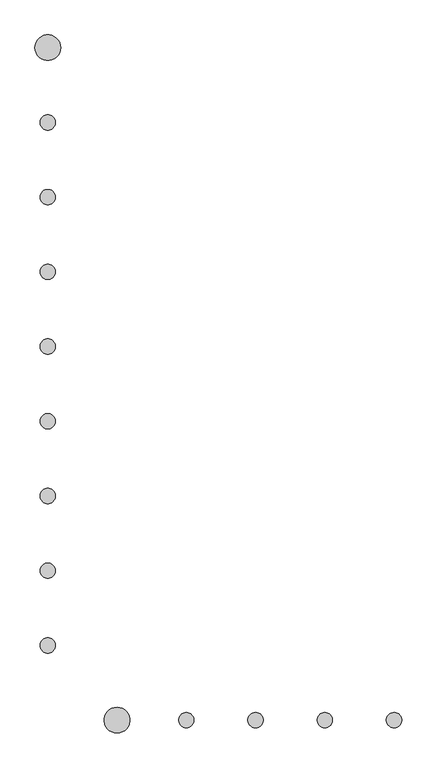
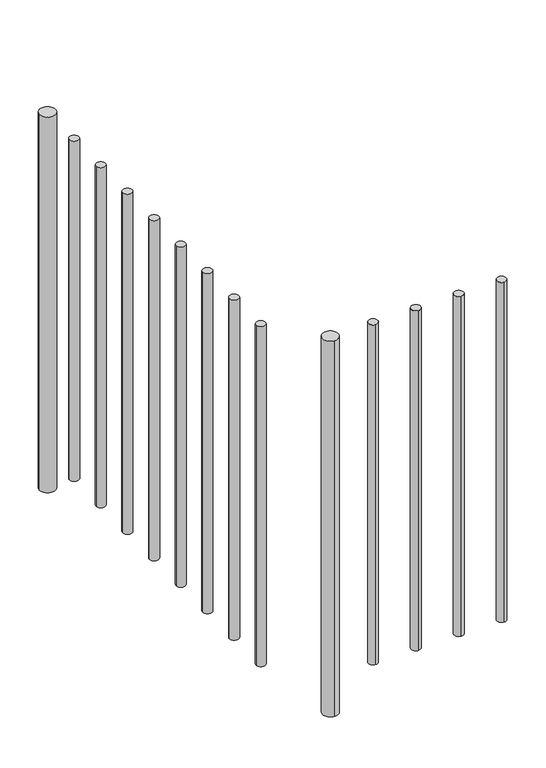
"""IFC4 building model written with IfcOpenShell, lengths in millimetres: railing geometry."""

from ifc_helpers import new_model, si_unit, point, frame, frame_2d, origin, place, context, project, spatial, circle_curve, trimmed, segment, composite_curve, outline, extrude, source, transform, mapped, element, save


def railing_35eac12f(model_context):
    return source(origin(), model_context, "Body", "SweptSolid", [
        extrude(outline(composite_curve([segment(trimmed(circle_curve(frame_2d((-2709.174449, -8163.7965465)), 12.5), [point((-2709.174449, -8176.2965465))], [point((-2709.174449, -8151.2965465))], False, "CARTESIAN"), True, "CONTINUOUS"), segment(trimmed(circle_curve(frame_2d((-2709.174449, -8163.7965465)), 12.5), [point((-2709.174449, -8151.2965465))], [point((-2709.174449, -8176.2965465))], False, "CARTESIAN"), True, "CONTINUOUS")], self_intersect=False)), frame((0.0, 0.0, 3500.0), z_axis=(0.0, 0.0, 1.0), x_axis=(1.0, 0.0, 0.0)), (0.0, 0.0, 1.0), 949.2),
        extrude(outline(composite_curve([segment(trimmed(circle_curve(frame_2d((-2822.314449, -8163.7965465)), 12.5), [point((-2822.314449, -8176.2965465))], [point((-2822.314449, -8151.2965465))], False, "CARTESIAN"), True, "CONTINUOUS"), segment(trimmed(circle_curve(frame_2d((-2822.314449, -8163.7965465)), 12.5), [point((-2822.314449, -8151.2965465))], [point((-2822.314449, -8176.2965465))], False, "CARTESIAN"), True, "CONTINUOUS")], self_intersect=False)), frame((0.0, 0.0, 3500.0), z_axis=(0.0, 0.0, 1.0), x_axis=(1.0, 0.0, 0.0)), (0.0, 0.0, 1.0), 949.2),
        extrude(outline(composite_curve([segment(trimmed(circle_curve(frame_2d((-2935.454449, -8163.7965465)), 12.5), [point((-2935.454449, -8176.2965465))], [point((-2935.454449, -8151.2965465))], False, "CARTESIAN"), True, "CONTINUOUS"), segment(trimmed(circle_curve(frame_2d((-2935.454449, -8163.7965465)), 12.5), [point((-2935.454449, -8151.2965465))], [point((-2935.454449, -8176.2965465))], False, "CARTESIAN"), True, "CONTINUOUS")], self_intersect=False)), frame((0.0, 0.0, 3500.0), z_axis=(0.0, 0.0, 1.0), x_axis=(1.0, 0.0, 0.0)), (0.0, 0.0, 1.0), 949.2),
        extrude(outline(composite_curve([segment(trimmed(circle_curve(frame_2d((-3048.594449, -8163.7965465)), 12.5), [point((-3048.594449, -8176.2965465))], [point((-3048.594449, -8151.2965465))], False, "CARTESIAN"), True, "CONTINUOUS"), segment(trimmed(circle_curve(frame_2d((-3048.594449, -8163.7965465)), 12.5), [point((-3048.594449, -8151.2965465))], [point((-3048.594449, -8176.2965465))], False, "CARTESIAN"), True, "CONTINUOUS")], self_intersect=False)), frame((0.0, 0.0, 3500.0), z_axis=(0.0, 0.0, 1.0), x_axis=(1.0, 0.0, 0.0)), (0.0, 0.0, 1.0), 949.2),
        extrude(outline(composite_curve([segment(trimmed(circle_curve(frame_2d((-3161.734449, -8163.7965465)), 21.0), [point((-3161.734449, -8184.7965465))], [point((-3161.734449, -8142.7965465))], False, "CARTESIAN"), True, "CONTINUOUS"), segment(trimmed(circle_curve(frame_2d((-3161.734449, -8163.7965465)), 21.0), [point((-3161.734449, -8142.7965465))], [point((-3161.734449, -8184.7965465))], False, "CARTESIAN"), True, "CONTINUOUS")], self_intersect=False)), frame((0.0, 0.0, 3400.0), z_axis=(0.0, 0.0, 1.0), x_axis=(1.0, 0.0, 0.0)), (0.0, 0.0, 1.0), 1049.2),
        extrude(outline(composite_curve([segment(trimmed(circle_curve(frame_2d((-3274.874449, -8041.7565465)), 12.5), [point((-3287.374449, -8041.7565465))], [point((-3262.374449, -8041.7565465))], False, "CARTESIAN"), True, "CONTINUOUS"), segment(trimmed(circle_curve(frame_2d((-3274.874449, -8041.7565465)), 12.5), [point((-3262.374449, -8041.7565465))], [point((-3287.374449, -8041.7565465))], False, "CARTESIAN"), True, "CONTINUOUS")], self_intersect=False)), frame((0.0, 0.0, 3500.0), z_axis=(0.0, 0.0, 1.0), x_axis=(1.0, 0.0, 0.0)), (0.0, 0.0, 1.0), 949.2),
        extrude(outline(composite_curve([segment(trimmed(circle_curve(frame_2d((-3274.874449, -7919.7165465)), 12.5), [point((-3287.374449, -7919.7165465))], [point((-3262.374449, -7919.7165465))], False, "CARTESIAN"), True, "CONTINUOUS"), segment(trimmed(circle_curve(frame_2d((-3274.874449, -7919.7165465)), 12.5), [point((-3262.374449, -7919.7165465))], [point((-3287.374449, -7919.7165465))], False, "CARTESIAN"), True, "CONTINUOUS")], self_intersect=False)), frame((0.0, 0.0, 3500.0), z_axis=(0.0, 0.0, 1.0), x_axis=(1.0, 0.0, 0.0)), (0.0, 0.0, 1.0), 949.2),
        extrude(outline(composite_curve([segment(trimmed(circle_curve(frame_2d((-3274.874449, -7797.6765465)), 12.5), [point((-3287.374449, -7797.6765465))], [point((-3262.374449, -7797.6765465))], False, "CARTESIAN"), True, "CONTINUOUS"), segment(trimmed(circle_curve(frame_2d((-3274.874449, -7797.6765465)), 12.5), [point((-3262.374449, -7797.6765465))], [point((-3287.374449, -7797.6765465))], False, "CARTESIAN"), True, "CONTINUOUS")], self_intersect=False)), frame((0.0, 0.0, 3500.0), z_axis=(0.0, 0.0, 1.0), x_axis=(1.0, 0.0, 0.0)), (0.0, 0.0, 1.0), 949.2),
        extrude(outline(composite_curve([segment(trimmed(circle_curve(frame_2d((-3274.874449, -7675.6365465)), 12.5), [point((-3287.374449, -7675.6365465))], [point((-3262.374449, -7675.6365465))], False, "CARTESIAN"), True, "CONTINUOUS"), segment(trimmed(circle_curve(frame_2d((-3274.874449, -7675.6365465)), 12.5), [point((-3262.374449, -7675.6365465))], [point((-3287.374449, -7675.6365465))], False, "CARTESIAN"), True, "CONTINUOUS")], self_intersect=False)), frame((0.0, 0.0, 3500.0), z_axis=(0.0, 0.0, 1.0), x_axis=(1.0, 0.0, 0.0)), (0.0, 0.0, 1.0), 949.2),
        extrude(outline(composite_curve([segment(trimmed(circle_curve(frame_2d((-3274.874449, -7553.5965465)), 12.5), [point((-3287.374449, -7553.5965465))], [point((-3262.374449, -7553.5965465))], False, "CARTESIAN"), True, "CONTINUOUS"), segment(trimmed(circle_curve(frame_2d((-3274.874449, -7553.5965465)), 12.5), [point((-3262.374449, -7553.5965465))], [point((-3287.374449, -7553.5965465))], False, "CARTESIAN"), True, "CONTINUOUS")], self_intersect=False)), frame((0.0, 0.0, 3500.0), z_axis=(0.0, 0.0, 1.0), x_axis=(1.0, 0.0, 0.0)), (0.0, 0.0, 1.0), 949.2),
        extrude(outline(composite_curve([segment(trimmed(circle_curve(frame_2d((-3274.874449, -7431.5565465)), 12.5), [point((-3287.374449, -7431.5565465))], [point((-3262.374449, -7431.5565465))], False, "CARTESIAN"), True, "CONTINUOUS"), segment(trimmed(circle_curve(frame_2d((-3274.874449, -7431.5565465)), 12.5), [point((-3262.374449, -7431.5565465))], [point((-3287.374449, -7431.5565465))], False, "CARTESIAN"), True, "CONTINUOUS")], self_intersect=False)), frame((0.0, 0.0, 3500.0), z_axis=(0.0, 0.0, 1.0), x_axis=(1.0, 0.0, 0.0)), (0.0, 0.0, 1.0), 949.2),
        extrude(outline(composite_curve([segment(trimmed(circle_curve(frame_2d((-3274.874449, -7309.5165465)), 12.5), [point((-3287.374449, -7309.5165465))], [point((-3262.374449, -7309.5165465))], False, "CARTESIAN"), True, "CONTINUOUS"), segment(trimmed(circle_curve(frame_2d((-3274.874449, -7309.5165465)), 12.5), [point((-3262.374449, -7309.5165465))], [point((-3287.374449, -7309.5165465))], False, "CARTESIAN"), True, "CONTINUOUS")], self_intersect=False)), frame((0.0, 0.0, 3500.0), z_axis=(0.0, 0.0, 1.0), x_axis=(1.0, 0.0, 0.0)), (0.0, 0.0, 1.0), 949.2),
        extrude(outline(composite_curve([segment(trimmed(circle_curve(frame_2d((-3274.874449, -7187.4765465)), 12.5), [point((-3287.374449, -7187.4765465))], [point((-3262.374449, -7187.4765465))], False, "CARTESIAN"), True, "CONTINUOUS"), segment(trimmed(circle_curve(frame_2d((-3274.874449, -7187.4765465)), 12.5), [point((-3262.374449, -7187.4765465))], [point((-3287.374449, -7187.4765465))], False, "CARTESIAN"), True, "CONTINUOUS")], self_intersect=False)), frame((0.0, 0.0, 3500.0), z_axis=(0.0, 0.0, 1.0), x_axis=(1.0, 0.0, 0.0)), (0.0, 0.0, 1.0), 949.2),
        extrude(outline(composite_curve([segment(trimmed(circle_curve(frame_2d((-3274.874449, -7065.4365465)), 21.0), [point((-3295.874449, -7065.4365465))], [point((-3253.874449, -7065.4365465))], False, "CARTESIAN"), True, "CONTINUOUS"), segment(trimmed(circle_curve(frame_2d((-3274.874449, -7065.4365465)), 21.0), [point((-3253.874449, -7065.4365465))], [point((-3295.874449, -7065.4365465))], False, "CARTESIAN"), True, "CONTINUOUS")], self_intersect=False)), frame((0.0, 0.0, 3400.0), z_axis=(0.0, 0.0, 1.0), x_axis=(1.0, 0.0, 0.0)), (0.0, 0.0, 1.0), 1049.2),
    ])


if __name__ == "__main__":
    model = new_model("IFC4")
    model_context = context("Model", 3, world=origin())
    ifc_project = project(units=[si_unit("LENGTHUNIT", "METRE", prefix="MILLI")], contexts=[model_context])
    site = spatial("IfcSite", under=ifc_project)
    building = spatial("IfcBuilding", under=site)
    placement = place(None, origin())
    railing_shape = railing_35eac12f(model_context)
    element("IfcRailing", 1, at=placement, inside=building, context=model_context, shape_type="MappedRepresentation", body=[
        mapped(railing_shape, transform((0.0, 0.0, 0.0), x_axis=(1.0, 0.0, 0.0), y_axis=(0.0, 1.0, 0.0), z_axis=(0.0, 0.0, 1.0))),
    ])
    save(model, "model.ifc")

# Revit data of these elements
# Element 1 (IfcRailing)
#   Materials on its faces: "Ferro - Pintura Esmalte"
# Materials
#   "Ferro - Pintura Esmalte": class "Pintura", colour RGB 255 255 255, transparency 0, Cost = 0
